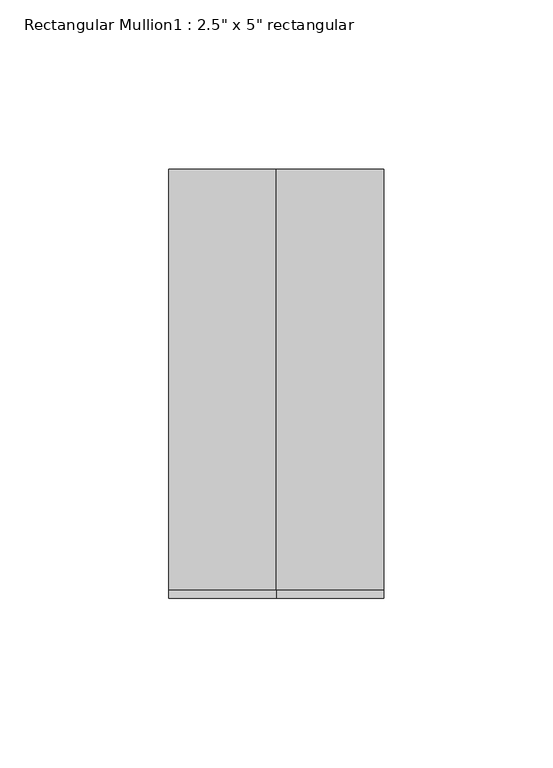
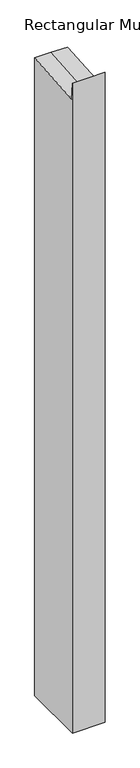
"""IFC4 building model written with IfcOpenShell, lengths in millimetres: member geometry."""

from ifc_helpers import new_model, si_unit, origin, place, context, project, spatial, faceted_brep, source, transform, mapped, element, save


def member_652a6926(model_context):
    return source(origin(), model_context, "Body", "Brep", [
        faceted_brep([(31.75, 63.5, -1302.7683735), (31.75, -63.5, -1302.7683735), (-31.75, -63.5, -1302.7683735), (-31.75, 63.5, -1302.7683735), (-31.75, 63.5, 4.512614), (0.0, 63.5, 4.512614), (31.75, 63.5, 4.512614), (-31.75, -63.5, 29.4551734), (-31.75, -61.0425175, -4.5008422), (31.75, -63.5, 29.4551734), (0.0, -63.5, 29.4551734), (31.75, -61.0425175, -4.5008422), (0.0, -61.0425175, -4.5008422)], [[[0, 1, 2, 3]], [[4, 5, 6, 0, 3]], [[7, 8, 4, 3, 2]], [[9, 10, 7, 2, 1]], [[6, 11, 9, 1, 0]], [[6, 5, 12, 11]], [[5, 4, 8, 12]], [[8, 7, 10, 12]], [[10, 9, 11, 12]]]),
    ])


if __name__ == "__main__":
    model = new_model("IFC4")
    model_context = context("Model", 3, world=origin())
    ifc_project = project(units=[si_unit("LENGTHUNIT", "METRE", prefix="MILLI")], contexts=[model_context])
    site = spatial("IfcSite", under=ifc_project)
    building = spatial("IfcBuilding", under=site)
    placement = place(None, origin())
    member_shape = member_652a6926(model_context)
    element("IfcMember", 1, ObjectType="Rectangular Mullion1 : 2.5\" x 5\" rectangular", at=placement, inside=building, context=model_context, shape_type="MappedRepresentation", body=[
        mapped(member_shape, transform((0.0, 0.0, 0.0), x_axis=(1.0, 0.0, 0.0), y_axis=(0.0, 1.0, 0.0), z_axis=(0.0, 0.0, 1.0))),
    ])
    save(model, "model.ifc")

# Revit data of these elements
# Type "Rectangular Mullion1 : 2.5\" x 5\" rectangular"
#   built-in parameter 1007304 = 0.416667 (stored number, unit not read)
#   built-in parameter 1007301 = 0.104167 (stored number, unit not read)
#   built-in parameter 1007300 = 0.104167 (stored number, unit not read)
# Element 1 (IfcMember, "Rectangular Mullion1 : 2.5\" x 5\" rectangular")
#   Materials on its faces: "support-frame"
# Materials
#   "support-frame": class "Unassigned", colour RGB 233 233 233, transparency 0, Cost = 0
